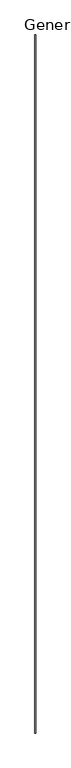
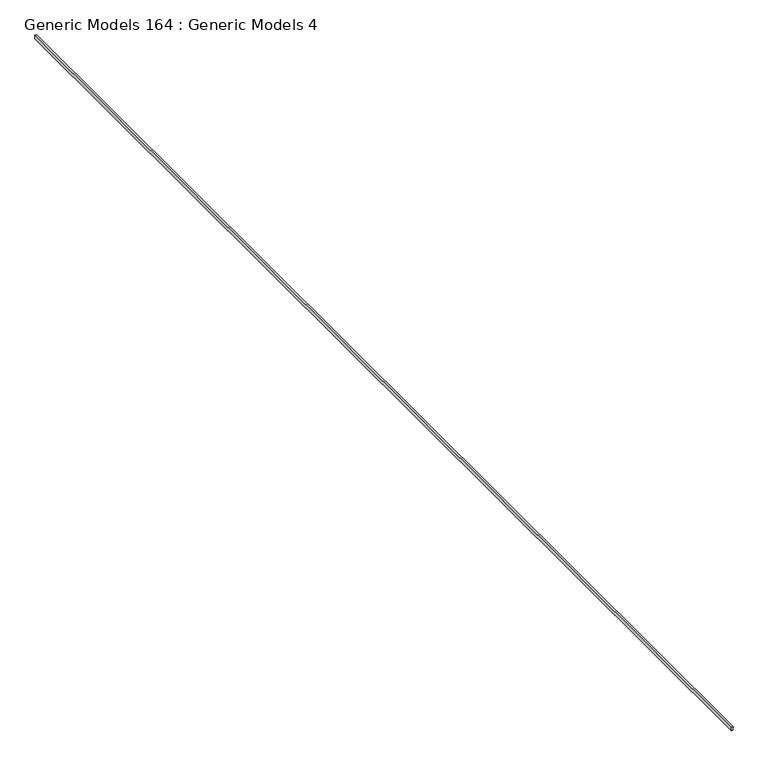
"""IFC4 building model written with IfcOpenShell, lengths in millimetres: proxy geometry, Generic Models 164 : Generic Models 4."""

from ifc_helpers import new_model, si_unit, origin, place, context, project, spatial, faceted_brep, source, transform, mapped, element, save


def generic_models_164_generic_models_4_104797f7(model_context):
    return source(origin(), model_context, "Body", "Brep", [
        faceted_brep([(-10252.9339552, -5493.3230338, 122820.8249647), (-10252.9339552, -5493.3230338, 122811.2999647), (-10252.9339552, -5493.3230338, 122784.1984874), (-10237.6972239, -5493.3230338, 122784.1984874), (-10237.6972239, -5493.3230338, 122811.2999647), (-10236.1097239, -5493.3230338, 122811.2999647), (-10236.1097239, -5493.3230338, 122820.8249647), (-10252.9339552, 7054.2769662, 122820.8249647), (-10236.1097239, 7054.2769662, 122820.8249647), (-10236.1097239, 7054.2769662, 122811.2999647), (-10237.6972239, 7054.2769662, 122811.2999647), (-10237.6972239, 7054.2769662, 122784.1984874), (-10252.9339552, 7054.2769662, 122784.1984874), (-10252.9339552, 7054.2769662, 122811.2999647)], [[[0, 1, 2, 3, 4, 5, 6]], [[7, 8, 9, 10, 11, 12, 13]], [[2, 1, 0, 7, 13, 12]], [[2, 12, 11, 3]], [[8, 6, 5, 9]], [[0, 6, 8, 7]], [[10, 4, 3, 11]], [[4, 10, 9, 5]]]),
    ])


if __name__ == "__main__":
    model = new_model("IFC4")
    model_context = context("Model", 3, world=origin())
    ifc_project = project(units=[si_unit("LENGTHUNIT", "METRE", prefix="MILLI")], contexts=[model_context])
    site = spatial("IfcSite", under=ifc_project)
    building = spatial("IfcBuilding", under=site)
    placement = place(None, origin())
    generic_models_164_generic_models_4_shape = generic_models_164_generic_models_4_104797f7(model_context)
    element("IfcBuildingElementProxy", 1, Name="Generic Models 164 : Generic Models 4", ObjectType="Generic Models 164 : Generic Models 4", at=placement, inside=building, context=model_context, shape_type="MappedRepresentation", body=[
        mapped(generic_models_164_generic_models_4_shape, transform((0.0, 0.0, 0.0), x_axis=(1.0, 0.0, 0.0), y_axis=(0.0, 1.0, 0.0), z_axis=(0.0, 0.0, 1.0))),
    ])
    save(model, "model.ifc")

# Revit data of these elements
# Element 1 (IfcBuildingElementProxy, "Generic Models 164 : Generic Models 4")
#   Materials on its faces: "_MORTAR SETTING BED"
# Materials
#   "_MORTAR SETTING BED": class "Generic", colour RGB 191 191 191, transparency 0, Cost = 0
